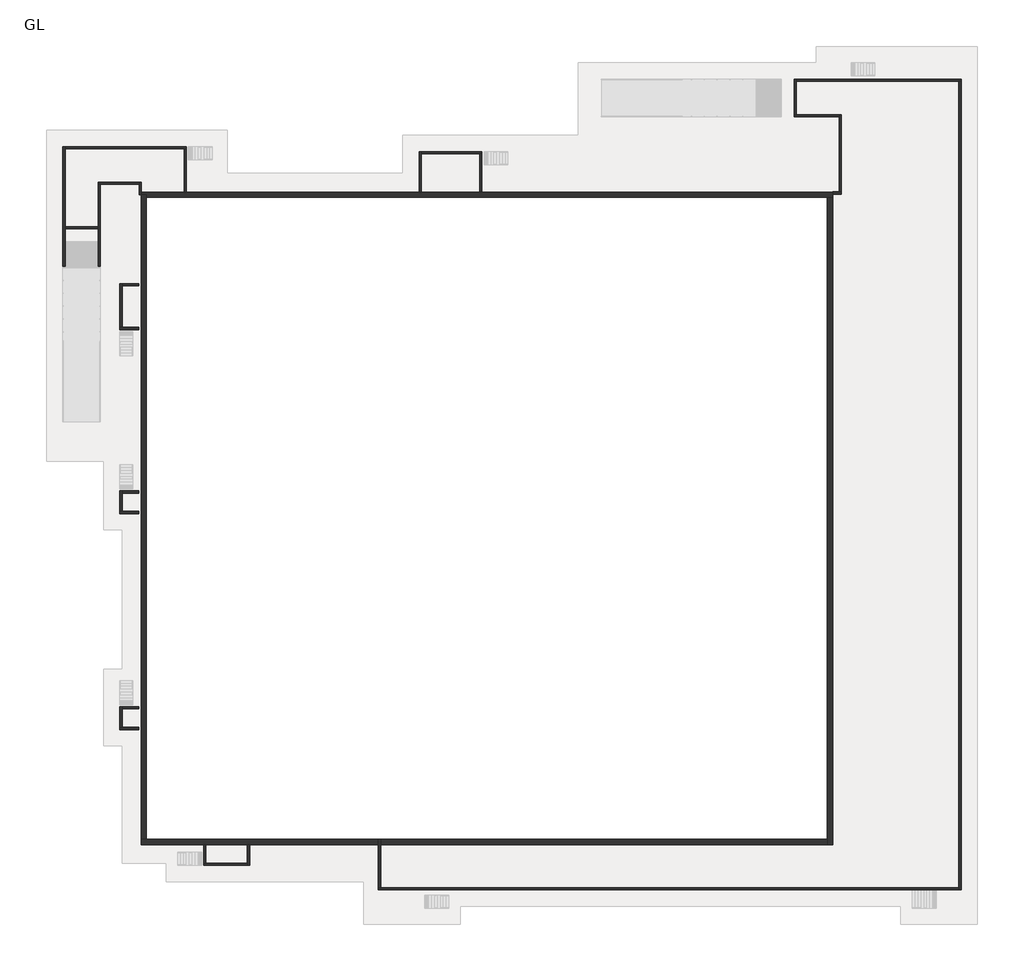
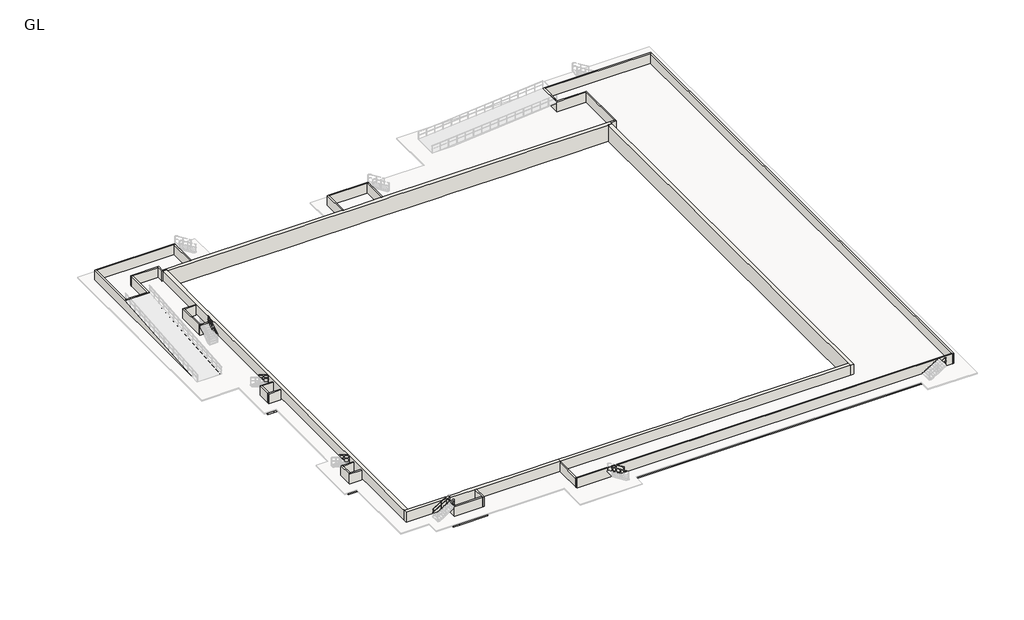
# One storey, part 1 of 2: 35 walls, 22 footings.
"""IFC4 building model written with IfcOpenShell, lengths in millimetres."""

from ifc_helpers import new_model, si_unit, frame, origin, place, context, project, spatial, polyline, outline, extrude, faceted_brep, element, save

model = new_model("IFC4")

# Units and contexts
model_context = context("Model", 3, world=origin())
ifc_project = project(units=[si_unit("LENGTHUNIT", "METRE", prefix="MILLI")], contexts=[model_context])

# Site, building, storey
site = spatial("IfcSite", under=ifc_project)
building = spatial("IfcBuilding", under=site)
storey = spatial("IfcBuildingStorey", under=building, Name="GL", Elevation=-1200.0)

# Footings
placement = place(None, origin())
element("IfcFooting", 1, ObjectType="900x300", at=placement, inside=storey, context=model_context, shape_type="Brep", body=[
    faceted_brep([(-450.0, 11324.7934796, -2200.0), (-450.0, 10424.7934796, -2200.0), (-450.0, 10424.7934796, -2500.0), (-450.0, 11324.7934796, -2500.0), (-1666.0, 11324.7934796, -2200.0), (-2566.0, 11324.7934796, -2200.0), (-2566.0, 10424.7934796, -2200.0), (-2566.0, 10424.7934796, -2500.0), (-2566.0, 11324.7934796, -2500.0), (-1666.0, 11324.7934796, -2500.0)], [[[0, 1, 2, 3]], [[0, 4, 5, 6, 1]], [[2, 1, 6, 7]], [[3, 2, 7, 8, 9]], [[0, 3, 9, 8, 5, 4]], [[6, 5, 8, 7]]]),
])
element("IfcFooting", 2, ObjectType="900x300", at=placement, inside=storey, context=model_context, shape_type="Brep", body=[
    faceted_brep([(-1666.0, 13262.7934796, -2200.0), (-2566.0, 13262.7934796, -2200.0), (-2566.0, 11324.7934796, -2200.0), (-1666.0, 11324.7934796, -2200.0), (-1666.0, 12362.7934796, -2200.0), (-2566.0, 13262.7934796, -2500.0), (-2566.0, 11324.7934796, -2500.0), (-1666.0, 13262.7934796, -2500.0), (-1666.0, 12362.7934796, -2500.0), (-1666.0, 11324.7934796, -2500.0)], [[[0, 1, 2, 3, 4]], [[1, 5, 6, 2]], [[5, 7, 8, 9, 6]], [[7, 0, 4, 3, 9, 8]], [[3, 2, 6, 9]], [[1, 0, 7, 5]]]),
])
element("IfcFooting", 3, ObjectType="900x300", at=placement, inside=storey, context=model_context, shape_type="SweptSolid", body=[
    extrude(outline(polyline([(-450.0, 13262.7934796), (-450.0, 12362.7934796), (-1666.0, 12362.7934796), (-1666.0, 13262.7934796), (-450.0, 13262.7934796)])), frame((0.0, 0.0, -2500.0), z_axis=(0.0, 0.0, 1.0), x_axis=(1.0, 0.0, 0.0)), (0.0, 0.0, 1.0), 300.0),
])
element("IfcFooting", 4, ObjectType="900x300", at=placement, inside=storey, context=model_context, shape_type="Brep", body=[
    faceted_brep([(5264.0, 47.0208589, -2200.0), (6164.0, 47.0208589, -2200.0), (6164.0, 47.0208589, -2500.0), (5264.0, 47.0208589, -2500.0), (6164.0, -2227.9791411, -2200.0), (6164.0, -1327.9791411, -2200.0), (5264.0, -2227.9791411, -2200.0), (5264.0, -2227.9791411, -2500.0), (6164.0, -2227.9791411, -2500.0), (6164.0, -1327.9791411, -2500.0)], [[[0, 1, 2, 3]], [[4, 5, 1, 0, 6]], [[7, 6, 0, 3]], [[8, 7, 3, 2, 9]], [[4, 8, 9, 2, 1, 5]], [[4, 6, 7, 8]]]),
])
element("IfcFooting", 5, ObjectType="900x300", at=placement, inside=storey, context=model_context, shape_type="Brep", body=[
    faceted_brep([(10234.5452414, -2227.9791411, -2200.0), (10234.5452414, -1327.9791411, -2200.0), (9334.5452414, -1327.9791411, -2200.0), (6164.0, -1327.9791411, -2200.0), (6164.0, -2227.9791411, -2200.0), (10234.5452414, -2227.9791411, -2500.0), (6164.0, -2227.9791411, -2500.0), (10234.5452414, -1327.9791411, -2500.0), (6164.0, -1327.9791411, -2500.0), (9334.5452414, -1327.9791411, -2500.0)], [[[0, 1, 2, 3, 4]], [[5, 0, 4, 6]], [[7, 5, 6, 8, 9]], [[1, 7, 9, 8, 3, 2]], [[4, 3, 8, 6]], [[1, 0, 5, 7]]]),
])
element("IfcFooting", 6, ObjectType="900x300", at=placement, inside=storey, context=model_context, shape_type="SweptSolid", body=[
    extrude(outline(polyline([(9334.5452414, 47.0208589), (10234.5452414, 47.0208589), (10234.5452414, -1327.9791411), (9334.5452414, -1327.9791411), (9334.5452414, 47.0208589)])), frame((0.0, 0.0, -2500.0), z_axis=(0.0, 0.0, 1.0), x_axis=(1.0, 0.0, 0.0)), (0.0, 0.0, 1.0), 300.0),
])
element("IfcFooting", 7, ObjectType="900x300", at=placement, inside=storey, context=model_context, shape_type="Brep", body=[
    faceted_brep([(21564.0, 547.0208589, -2200.0), (22464.0, 547.0208589, -2200.0), (22464.0, 547.0208589, -2500.0), (21564.0, 547.0208589, -2500.0), (22464.0, -4527.9791411, -2200.0), (22464.0, -3627.9791411, -2200.0), (21564.0, -4527.9791411, -2200.0), (21564.0, -4527.9791411, -2500.0), (22464.0, -4527.9791411, -2500.0), (22464.0, -3627.9791411, -2500.0)], [[[0, 1, 2, 3]], [[4, 5, 1, 0, 6]], [[7, 6, 0, 3]], [[8, 7, 3, 2, 9]], [[4, 8, 9, 2, 1, 5]], [[4, 6, 7, 8]]]),
])
element("IfcFooting", 8, ObjectType="900x300", at=placement, inside=storey, context=model_context, shape_type="Brep", body=[
    faceted_brep([(76641.0, -4527.9791411, -2200.0), (76641.0, -3627.9791411, -2200.0), (75741.0, -3627.9791411, -2200.0), (22464.0, -3627.9791411, -2200.0), (22464.0, -4527.9791411, -2200.0), (76641.0, -4527.9791411, -2500.0), (22464.0, -4527.9791411, -2500.0), (76641.0, -3627.9791411, -2500.0), (22464.0, -3627.9791411, -2500.0), (75741.0, -3627.9791411, -2500.0)], [[[0, 1, 2, 3, 4]], [[5, 0, 4, 6]], [[7, 5, 6, 8, 9]], [[1, 7, 9, 8, 3, 2]], [[4, 3, 8, 6]], [[1, 0, 5, 7]]]),
])
element("IfcFooting", 9, ObjectType="900x300", at=placement, inside=storey, context=model_context, shape_type="SweptSolid", body=[
    extrude(outline(polyline([(26250.0, 60949.5208589), (25350.0, 60949.5208589), (25350.0, 64152.0208589), (26250.0, 64152.0208589), (26250.0, 60949.5208589)])), frame((0.0, 0.0, -2500.0), z_axis=(0.0, 0.0, 1.0), x_axis=(1.0, 0.0, 0.0)), (0.0, 0.0, 1.0), 300.0),
])
element("IfcFooting", 10, ObjectType="900x300", at=placement, inside=storey, context=model_context, shape_type="Brep", body=[
    faceted_brep([(4325.7243044, 60949.5208589, -2200.0), (3425.7243044, 60949.5208589, -2200.0), (3425.7243044, 60949.5208589, -2500.0), (4325.7243044, 60949.5208589, -2500.0), (3425.7243044, 65527.0208589, -2200.0), (3425.7243044, 64627.0208589, -2200.0), (4325.7243044, 65527.0208589, -2200.0), (4325.7243044, 65527.0208589, -2500.0), (3425.7243044, 65527.0208589, -2500.0), (3425.7243044, 64627.0208589, -2500.0)], [[[0, 1, 2, 3]], [[4, 5, 1, 0, 6]], [[7, 6, 0, 3]], [[8, 7, 3, 2, 9]], [[4, 8, 9, 2, 1, 5]], [[4, 6, 7, 8]]]),
])
element("IfcFooting", 11, ObjectType="900x300", at=placement, inside=storey, context=model_context, shape_type="Brep", body=[
    faceted_brep([(132.1872592, 60699.5208589, -2200.0), (-767.8127408, 60699.5208589, -2200.0), (-767.8127408, 60699.5208589, -2500.0), (132.1872592, 60699.5208589, -2500.0), (132.1872592, 62227.0208589, -2200.0), (-767.8127408, 62227.0208589, -2200.0), (-767.8127408, 61327.0208589, -2200.0), (-767.8127408, 62227.0208589, -2500.0), (-767.8127408, 61327.0208589, -2500.0), (132.1872592, 62227.0208589, -2500.0)], [[[0, 1, 2, 3]], [[0, 4, 5, 6, 1]], [[2, 1, 6, 5, 7, 8]], [[3, 2, 8, 7, 9]], [[0, 3, 9, 4]], [[5, 4, 9, 7]]]),
])
element("IfcFooting", 12, ObjectType="900x300", at=placement, inside=storey, context=model_context, shape_type="Brep", body=[
    faceted_brep([(-4591.0, 62227.0208589, -2200.0), (-4591.0, 61327.0208589, -2200.0), (-3691.0, 61327.0208589, -2200.0), (-767.8127408, 61327.0208589, -2200.0), (-767.8127408, 62227.0208589, -2200.0), (-4591.0, 61327.0208589, -2500.0), (-3691.0, 61327.0208589, -2500.0), (-767.8127408, 61327.0208589, -2500.0), (-4591.0, 62227.0208589, -2500.0), (-767.8127408, 62227.0208589, -2500.0)], [[[0, 1, 2, 3, 4]], [[1, 5, 6, 7, 3, 2]], [[5, 8, 9, 7, 6]], [[8, 0, 4, 9]], [[4, 3, 7, 9]], [[1, 0, 8, 5]]]),
])
element("IfcFooting", 13, ObjectType="900x300", at=placement, inside=storey, context=model_context, shape_type="SweptSolid", body=[
    extrude(outline(polyline([(-7891.0, 64627.0208589), (-7891.0, 65527.0208589), (3425.7243044, 65527.0208589), (3425.7243044, 64627.0208589), (-7891.0, 64627.0208589)])), frame((0.0, 0.0, -2500.0), z_axis=(0.0, 0.0, 1.0), x_axis=(1.0, 0.0, 0.0)), (0.0, 0.0, 1.0), 300.0),
])
element("IfcFooting", 14, ObjectType="900x300", at=placement, inside=storey, context=model_context, shape_type="Brep", body=[
    faceted_brep([(-3691.0, 39561.4815956, -2500.0), (-3691.0, 39561.4815956, -2200.0), (-4591.0, 39561.4815956, -2200.0), (-4591.0, 39561.4815956, -2500.0), (-3691.0, 61327.0208589, -2200.0), (-4591.0, 61327.0208589, -2200.0), (-4591.0, 58048.9598198, -2200.0), (-4591.0, 57148.9598198, -2200.0), (-3691.0, 61327.0208589, -2500.0), (-4591.0, 57148.9598198, -2500.0), (-4591.0, 58048.9598198, -2500.0), (-4591.0, 61327.0208589, -2500.0)], [[[0, 1, 2, 3]], [[2, 1, 4, 5, 6, 7]], [[1, 0, 8, 4]], [[0, 3, 9, 10, 11, 8]], [[3, 2, 7, 6, 5, 11, 10, 9]], [[5, 4, 8, 11]]]),
])
element("IfcFooting", 15, ObjectType="900x300", at=placement, inside=storey, context=model_context, shape_type="Brep", body=[
    faceted_brep([(-6991.0, 39498.9598199, -2200.0), (-7891.0, 39498.9598199, -2200.0), (-7891.0, 39498.9598199, -2500.0), (-6991.0, 39498.9598199, -2500.0), (-6991.0, 57148.9598198, -2200.0), (-6991.0, 58048.9598198, -2200.0), (-6991.0, 64627.0208589, -2200.0), (-7891.0, 65527.0208589, -2200.0), (-7891.0, 65527.0208589, -2500.0), (-6991.0, 64627.0208589, -2500.0), (-6991.0, 58048.9598198, -2500.0), (-6991.0, 57148.9598198, -2500.0)], [[[0, 1, 2, 3]], [[0, 4, 5, 6, 7, 1]], [[2, 1, 7, 8]], [[3, 2, 8, 9, 10, 11]], [[0, 3, 11, 10, 9, 6, 5, 4]], [[7, 6, 9, 8]]]),
    faceted_brep([(-6991.0, 39677.0208589, -2200.0), (-7891.0, 39677.0208589, -2200.0), (-7891.0, 39677.0208589, -2500.0), (-6991.0, 39677.0208589, -2500.0), (-6991.0, 57148.9598198, -2200.0), (-6991.0, 58048.9598198, -2200.0), (-6991.0, 65527.0208589, -2200.0), (-7891.0, 65527.0208589, -2200.0), (-7891.0, 65527.0208589, -2500.0), (-6991.0, 65527.0208589, -2500.0), (-6991.0, 58048.9598198, -2500.0), (-6991.0, 57148.9598198, -2500.0)], [[[0, 1, 2, 3]], [[0, 4, 5, 6, 7, 1]], [[2, 1, 7, 8]], [[3, 2, 8, 9, 10, 11]], [[0, 3, 11, 10, 9, 6, 5, 4]], [[7, 6, 9, 8]]]),
])
element("IfcFooting", 16, ObjectType="900x300", at=placement, inside=storey, context=model_context, shape_type="SweptSolid", body=[
    extrude(outline(polyline([(-4591.0, 58048.9598198), (-4591.0, 57148.9598198), (-6991.0, 57148.9598198), (-6991.0, 58048.9598198), (-4591.0, 58048.9598198)])), frame((0.0, 0.0, -2500.0), z_axis=(0.0, 0.0, 1.0), x_axis=(1.0, 0.0, 0.0)), (0.0, 0.0, 1.0), 300.0),
])
element("IfcFooting", 17, ObjectType="900x300", at=placement, inside=storey, context=model_context, shape_type="Brep", body=[
    faceted_brep([(-450.0, 52734.7934796, -2200.0), (-450.0, 51834.7934796, -2200.0), (-450.0, 51834.7934796, -2500.0), (-450.0, 52734.7934796, -2500.0), (-2566.0, 51834.7934796, -2200.0), (-1666.0, 51834.7934796, -2200.0), (-2566.0, 52734.7934796, -2200.0), (-2566.0, 52734.7934796, -2500.0), (-2566.0, 51834.7934796, -2500.0), (-1666.0, 51834.7934796, -2500.0)], [[[0, 1, 2, 3]], [[4, 5, 1, 0, 6]], [[7, 6, 0, 3]], [[8, 7, 3, 2, 9]], [[4, 8, 9, 2, 1, 5]], [[4, 6, 7, 8]]]),
])
element("IfcFooting", 18, ObjectType="900x300", at=placement, inside=storey, context=model_context, shape_type="Brep", body=[
    faceted_brep([(-2566.0, 47764.2482382, -2200.0), (-1666.0, 47764.2482382, -2200.0), (-1666.0, 48664.2482382, -2200.0), (-1666.0, 51834.7934796, -2200.0), (-2566.0, 51834.7934796, -2200.0), (-2566.0, 47764.2482382, -2500.0), (-2566.0, 51834.7934796, -2500.0), (-1666.0, 47764.2482382, -2500.0), (-1666.0, 51834.7934796, -2500.0), (-1666.0, 48664.2482382, -2500.0)], [[[0, 1, 2, 3, 4]], [[5, 0, 4, 6]], [[7, 5, 6, 8, 9]], [[1, 7, 9, 8, 3, 2]], [[4, 3, 8, 6]], [[1, 0, 5, 7]]]),
])
element("IfcFooting", 19, ObjectType="900x300", at=placement, inside=storey, context=model_context, shape_type="SweptSolid", body=[
    extrude(outline(polyline([(-450.0, 48664.2482382), (-450.0, 47764.2482382), (-1666.0, 47764.2482382), (-1666.0, 48664.2482382), (-450.0, 48664.2482382)])), frame((0.0, 0.0, -2500.0), z_axis=(0.0, 0.0, 1.0), x_axis=(1.0, 0.0, 0.0)), (0.0, 0.0, 1.0), 300.0),
])
element("IfcFooting", 20, ObjectType="900x300", at=placement, inside=storey, context=model_context, shape_type="Brep", body=[
    faceted_brep([(-450.0, 33396.2934796, -2200.0), (-450.0, 32496.2934796, -2200.0), (-450.0, 32496.2934796, -2500.0), (-450.0, 33396.2934796, -2500.0), (-2566.0, 32496.2934796, -2200.0), (-1666.0, 32496.2934796, -2200.0), (-2566.0, 33396.2934796, -2200.0), (-2566.0, 33396.2934796, -2500.0), (-2566.0, 32496.2934796, -2500.0), (-1666.0, 32496.2934796, -2500.0)], [[[0, 1, 2, 3]], [[4, 5, 1, 0, 6]], [[7, 6, 0, 3]], [[8, 7, 3, 2, 9]], [[4, 8, 9, 2, 1, 5]], [[4, 6, 7, 8]]]),
])
element("IfcFooting", 21, ObjectType="900x300", at=placement, inside=storey, context=model_context, shape_type="Brep", body=[
    faceted_brep([(-2566.0, 30586.2934796, -2200.0), (-1666.0, 30586.2934796, -2200.0), (-1666.0, 31486.2934796, -2200.0), (-1666.0, 32496.2934796, -2200.0), (-2566.0, 32496.2934796, -2200.0), (-2566.0, 30586.2934796, -2500.0), (-2566.0, 32496.2934796, -2500.0), (-1666.0, 30586.2934796, -2500.0), (-1666.0, 32496.2934796, -2500.0), (-1666.0, 31486.2934796, -2500.0)], [[[0, 1, 2, 3, 4]], [[5, 0, 4, 6]], [[7, 5, 6, 8, 9]], [[1, 7, 9, 8, 3, 2]], [[4, 3, 8, 6]], [[1, 0, 5, 7]]]),
])
element("IfcFooting", 22, ObjectType="900x300", at=placement, inside=storey, context=model_context, shape_type="SweptSolid", body=[
    extrude(outline(polyline([(-450.0, 31486.2934796), (-450.0, 30586.2934796), (-1666.0, 30586.2934796), (-1666.0, 31486.2934796), (-450.0, 31486.2934796)])), frame((0.0, 0.0, -2500.0), z_axis=(0.0, 0.0, 1.0), x_axis=(1.0, 0.0, 0.0)), (0.0, 0.0, 1.0), 300.0),
])

# Walls
element("IfcWall", 23, ObjectType="H_WA_AMW_RC Wall_T200 (No Finish)", at=placement, inside=storey, context=model_context, shape_type="Brep", body=[
    faceted_brep([(64291.0, 60752.0208589, -2200.0), (65094.3815191, 60752.0208589, -2200.0), (65094.3815191, 60752.0208589, 300.0), (64291.0, 60752.0208589, 300.0), (64291.0, 60952.0208589, -2200.0), (64291.0, 60952.0208589, 300.0), (64894.3815191, 60952.0208589, 300.0), (65094.3815191, 60952.0208589, 300.0), (65094.3815191, 60952.0208589, -2200.0), (64894.3815191, 60952.0208589, -2200.0), (64291.0, 60949.5208589, -2200.0), (64291.0, 60949.5208589, 300.0)], [[[0, 1, 2, 3]], [[4, 5, 6, 7, 8, 9]], [[1, 0, 10, 4, 9, 8]], [[3, 2, 7, 6, 5, 11]], [[2, 1, 8, 7]], [[0, 3, 11, 5, 4, 10]]]),
])
element("IfcWall", 24, ObjectType="H_WA_AMW_RC Wall_T200 (No Finish)", at=placement, inside=storey, context=model_context, shape_type="Brep", body=[
    faceted_brep([(65094.3815191, 60952.0208589, -2200.0), (65094.3815191, 68177.0208589, -2200.0), (65094.3815191, 68177.0208589, 300.0), (65094.3815191, 60952.0208589, 300.0), (64894.3815191, 60952.0208589, -2200.0), (64894.3815191, 60952.0208589, 300.0), (64894.3815191, 67977.0208589, 300.0), (64894.3815191, 68177.0208589, 300.0), (64894.3815191, 68177.0208589, -2200.0), (64894.3815191, 67977.0208589, -2200.0)], [[[0, 1, 2, 3]], [[4, 5, 6, 7, 8, 9]], [[1, 0, 4, 9, 8]], [[3, 2, 7, 6, 5]], [[0, 3, 5, 4]], [[2, 1, 8, 7]]]),
])
element("IfcWall", 25, ObjectType="H_WA_AMW_RC Wall_T200 (No Finish)", at=placement, inside=storey, context=model_context, shape_type="Brep", body=[
    faceted_brep([(64894.3815191, 68177.0208589, -2200.0), (60916.32048, 68177.0208589, -2200.0), (60716.32048, 68177.0208589, -2200.0), (60716.32048, 68177.0208589, 300.0), (60916.32048, 68177.0208589, 300.0), (64894.3815191, 68177.0208589, 300.0), (64894.3815191, 67977.0208589, -2200.0), (64894.3815191, 67977.0208589, 300.0), (60716.32048, 67977.0208589, 300.0), (60716.32048, 67977.0208589, -2200.0)], [[[0, 1, 2, 3, 4, 5]], [[6, 7, 8, 9]], [[2, 1, 0, 6, 9]], [[5, 4, 3, 8, 7]], [[0, 5, 7, 6]], [[3, 2, 9, 8]]]),
])
element("IfcWall", 26, ObjectType="H_WA_AMW_RC Wall_T200 (No Finish)", at=placement, inside=storey, context=model_context, shape_type="Brep", body=[
    faceted_brep([(60916.32048, 68177.0208589, -2200.0), (60916.32048, 71277.0208589, -2200.0), (60916.32048, 71477.0208589, -2200.0), (60916.32048, 71477.0208589, 300.0), (60916.32048, 71277.0208589, 300.0), (60916.32048, 68177.0208589, 300.0), (60716.32048, 68177.0208589, -2200.0), (60716.32048, 68177.0208589, 300.0), (60716.32048, 71477.0208589, 300.0), (60716.32048, 71477.0208589, -2200.0)], [[[0, 1, 2, 3, 4, 5]], [[6, 7, 8, 9]], [[2, 1, 0, 6, 9]], [[5, 4, 3, 8, 7]], [[0, 5, 7, 6]], [[3, 2, 9, 8]]]),
])
element("IfcWall", 27, ObjectType="H_WA_AMW_RC Wall_T200 (No Finish)", at=placement, inside=storey, context=model_context, shape_type="Brep", body=[
    faceted_brep([(60916.32048, 71277.0208589, -2200.0), (76091.0, 71277.0208589, -2200.0), (76291.0, 71277.0208589, -2200.0), (76291.0, 71277.0208589, 300.0), (76091.0, 71277.0208589, 300.0), (60916.32048, 71277.0208589, 300.0), (60916.32048, 71477.0208589, -2200.0), (60916.32048, 71477.0208589, 300.0), (76291.0, 71477.0208589, 300.0), (76291.0, 71477.0208589, -2200.0)], [[[0, 1, 2, 3, 4, 5]], [[6, 7, 8, 9]], [[2, 1, 0, 6, 9]], [[5, 4, 3, 8, 7]], [[0, 5, 7, 6]], [[3, 2, 9, 8]]]),
])
element("IfcWall", 28, ObjectType="H_WA_AMW_RC Wall_T200 (No Finish)", at=placement, inside=storey, context=model_context, shape_type="Brep", body=[
    faceted_brep([(76091.0, 71277.0208589, -2200.0), (76091.0, -3977.9791411, -2200.0), (76091.0, -4177.9791411, -2200.0), (76091.0, -4177.9791411, 300.0), (76091.0, -3977.9791411, 300.0), (76091.0, 71277.0208589, 300.0), (76291.0, 71277.0208589, -2200.0), (76291.0, 71277.0208589, 300.0), (76291.0, -4177.9791411, 300.0), (76291.0, -4177.9791411, -2200.0)], [[[0, 1, 2, 3, 4, 5]], [[6, 7, 8, 9]], [[2, 1, 0, 6, 9]], [[5, 4, 3, 8, 7]], [[0, 5, 7, 6]], [[3, 2, 9, 8]]]),
])
element("IfcWall", 29, ObjectType="H_WA_AMW_RC Wall_T200 (No Finish)", at=placement, inside=storey, context=model_context, shape_type="Brep", body=[
    faceted_brep([(76091.0, -3977.9791411, -2200.0), (22114.0, -3977.9791411, -2200.0), (21914.0, -3977.9791411, -2200.0), (21914.0, -3977.9791411, 150.0), (21914.0, -3977.9791411, 300.0), (76091.0, -3977.9791411, 300.0), (76091.0, -4177.9791411, -2200.0), (76091.0, -4177.9791411, 300.0), (21914.0, -4177.9791411, 300.0), (21914.0, -4177.9791411, -2200.0)], [[[0, 1, 2, 3, 4, 5]], [[6, 7, 8, 9]], [[2, 1, 0, 6, 9]], [[5, 4, 8, 7]], [[4, 3, 2, 9, 8]], [[0, 5, 7, 6]]]),
])
element("IfcWall", 30, ObjectType="H_WA_AMW_RC Wall_T200 (No Finish)", at=placement, inside=storey, context=model_context, shape_type="Brep", body=[
    faceted_brep([(22114.0, -3977.9791411, -2200.0), (22114.0, 49.5208589, -2200.0), (22114.0, 547.0208589, -2200.0), (22114.0, 547.0208589, 150.0), (22114.0, 49.5208589, 150.0), (22114.0, -3977.9791411, 150.0), (21914.0, -3977.9791411, -2200.0), (21914.0, -3977.9791411, 150.0), (21914.0, 47.0208589, 150.0), (21914.0, 547.0208589, 150.0), (21914.0, 547.0208589, -2200.0), (21914.0, 47.0208589, -2200.0), (22014.0, 547.0208589, 150.0)], [[[0, 1, 2, 3, 4, 5]], [[6, 7, 8, 9, 10, 11]], [[2, 1, 0, 6, 11, 10]], [[5, 4, 3, 12, 9, 8, 7]], [[0, 5, 7, 6]], [[3, 2, 10, 9, 12]]]),
])
element("IfcWall", 31, ObjectType="H_WA_AMW_RC Wall_T200 (No Finish)", at=placement, inside=storey, context=model_context, shape_type="Brep", body=[
    faceted_brep([(9684.5452414, 47.0208589, -2200.0), (9684.5452414, -1677.9791411, -2200.0), (9684.5452414, -1877.9791411, -2200.0), (9684.5452414, -1877.9791411, 300.0), (9684.5452414, -1677.9791411, 300.0), (9684.5452414, 47.0208589, 300.0), (9884.5452414, 47.0208589, -2200.0), (9884.5452414, 47.0208589, 300.0), (9884.5452414, -1877.9791411, 300.0), (9884.5452414, -1877.9791411, -2200.0)], [[[0, 1, 2, 3, 4, 5]], [[6, 7, 8, 9]], [[2, 1, 0, 6, 9]], [[5, 4, 3, 8, 7]], [[3, 2, 9, 8]], [[0, 5, 7, 6]]]),
])
element("IfcWall", 32, ObjectType="H_WA_AMW_RC Wall_T200 (No Finish)", at=placement, inside=storey, context=model_context, shape_type="Brep", body=[
    faceted_brep([(9684.5452414, -1677.9791411, -2200.0), (5814.0, -1677.9791411, -2200.0), (5614.0, -1677.9791411, -2200.0), (5614.0, -1677.9791411, 300.0), (5814.0, -1677.9791411, 300.0), (9684.5452414, -1677.9791411, 300.0), (9684.5452414, -1877.9791411, -2200.0), (9684.5452414, -1877.9791411, 300.0), (5614.0, -1877.9791411, 300.0), (5614.0, -1877.9791411, -2200.0)], [[[0, 1, 2, 3, 4, 5]], [[6, 7, 8, 9]], [[2, 1, 0, 6, 9]], [[5, 4, 3, 8, 7]], [[0, 5, 7, 6]], [[3, 2, 9, 8]]]),
])
element("IfcWall", 33, ObjectType="H_WA_AMW_RC Wall_T200 (No Finish)", at=placement, inside=storey, context=model_context, shape_type="SweptSolid", body=[
    extrude(outline(polyline([(5814.0, 47.0208589), (5814.0, -1677.9791411), (5614.0, -1677.9791411), (5614.0, 47.0208589), (5814.0, 47.0208589)])), frame((0.0, 0.0, -2200.0), z_axis=(0.0, 0.0, 1.0), x_axis=(1.0, 0.0, 0.0)), (0.0, 0.0, 1.0), 2500.0),
])
element("IfcWall", 34, ObjectType="H_WA_AMW_RC Wall_T200 (No Finish)", at=placement, inside=storey, context=model_context, shape_type="Brep", body=[
    faceted_brep([(-450.0, 10974.7934796, -2200.0), (-2016.0, 10974.7934796, -2200.0), (-2216.0, 10974.7934796, -2200.0), (-2216.0, 10974.7934796, 300.0), (-2016.0, 10974.7934796, 300.0), (-450.0, 10974.7934796, 300.0), (-450.0, 10774.7934796, -2200.0), (-450.0, 10774.7934796, 300.0), (-2216.0, 10774.7934796, 300.0), (-2216.0, 10774.7934796, -2200.0)], [[[0, 1, 2, 3, 4, 5]], [[6, 7, 8, 9]], [[2, 1, 0, 6, 9]], [[5, 4, 3, 8, 7]], [[0, 5, 7, 6]], [[3, 2, 9, 8]]]),
])
element("IfcWall", 35, ObjectType="H_WA_AMW_RC Wall_T200 (No Finish)", at=placement, inside=storey, context=model_context, shape_type="Brep", body=[
    faceted_brep([(-2016.0, 10974.7934796, -2200.0), (-2016.0, 12712.7934796, -2200.0), (-2016.0, 12912.7934796, -2200.0), (-2016.0, 12912.7934796, 300.0), (-2016.0, 12712.7934796, 300.0), (-2016.0, 10974.7934796, 300.0), (-2216.0, 10974.7934796, -2200.0), (-2216.0, 10974.7934796, 300.0), (-2216.0, 12912.7934796, 300.0), (-2216.0, 12912.7934796, -2200.0)], [[[0, 1, 2, 3, 4, 5]], [[6, 7, 8, 9]], [[2, 1, 0, 6, 9]], [[5, 4, 3, 8, 7]], [[0, 5, 7, 6]], [[3, 2, 9, 8]]]),
])
element("IfcWall", 36, ObjectType="H_WA_AMW_RC Wall_T200 (No Finish)", at=placement, inside=storey, context=model_context, shape_type="SweptSolid", body=[
    extrude(outline(polyline([(-450.0, 12712.7934796), (-2016.0, 12712.7934796), (-2016.0, 12912.7934796), (-450.0, 12912.7934796), (-450.0, 12712.7934796)])), frame((0.0, 0.0, -2200.0), z_axis=(0.0, 0.0, 1.0), x_axis=(1.0, 0.0, 0.0)), (0.0, 0.0, 1.0), 2500.0),
])
element("IfcWall", 37, ObjectType="H_WA_AMW_RC Wall_T200 (No Finish)", at=placement, inside=storey, context=model_context, shape_type="Brep", body=[
    faceted_brep([(-450.0, 31136.2934796, -2200.0), (-2016.0, 31136.2934796, -2200.0), (-2216.0, 31136.2934796, -2200.0), (-2216.0, 31136.2934796, 300.0), (-2016.0, 31136.2934796, 300.0), (-450.0, 31136.2934796, 300.0), (-450.0, 30936.2934796, -2200.0), (-450.0, 30936.2934796, 300.0), (-2216.0, 30936.2934796, 300.0), (-2216.0, 30936.2934796, -2200.0)], [[[0, 1, 2, 3, 4, 5]], [[6, 7, 8, 9]], [[2, 1, 0, 6, 9]], [[5, 4, 3, 8, 7]], [[0, 5, 7, 6]], [[3, 2, 9, 8]]]),
])
element("IfcWall", 38, ObjectType="H_WA_AMW_RC Wall_T200 (No Finish)", at=placement, inside=storey, context=model_context, shape_type="Brep", body=[
    faceted_brep([(-2016.0, 31136.2934796, -2200.0), (-2016.0, 32846.2934796, -2200.0), (-2016.0, 33046.2934796, -2200.0), (-2016.0, 33046.2934796, 300.0), (-2016.0, 32846.2934796, 300.0), (-2016.0, 31136.2934796, 300.0), (-2216.0, 31136.2934796, -2200.0), (-2216.0, 31136.2934796, 300.0), (-2216.0, 33046.2934796, 300.0), (-2216.0, 33046.2934796, -2200.0)], [[[0, 1, 2, 3, 4, 5]], [[6, 7, 8, 9]], [[2, 1, 0, 6, 9]], [[5, 4, 3, 8, 7]], [[0, 5, 7, 6]], [[3, 2, 9, 8]]]),
])
element("IfcWall", 39, ObjectType="H_WA_AMW_RC Wall_T200 (No Finish)", at=placement, inside=storey, context=model_context, shape_type="SweptSolid", body=[
    extrude(outline(polyline([(-450.0, 32846.2934796), (-2016.0, 32846.2934796), (-2016.0, 33046.2934796), (-450.0, 33046.2934796), (-450.0, 32846.2934796)])), frame((0.0, 0.0, -2200.0), z_axis=(0.0, 0.0, 1.0), x_axis=(1.0, 0.0, 0.0)), (0.0, 0.0, 1.0), 2500.0),
])
element("IfcWall", 40, ObjectType="H_WA_AMW_RC Wall_T200 (No Finish)", at=placement, inside=storey, context=model_context, shape_type="Brep", body=[
    faceted_brep([(-450.0, 48314.2482382, -2200.0), (-2016.0, 48314.2482382, -2200.0), (-2216.0, 48314.2482382, -2200.0), (-2216.0, 48314.2482382, 300.0), (-2016.0, 48314.2482382, 300.0), (-450.0, 48314.2482382, 300.0), (-450.0, 48114.2482382, -2200.0), (-450.0, 48114.2482382, 300.0), (-2216.0, 48114.2482382, 300.0), (-2216.0, 48114.2482382, -2200.0)], [[[0, 1, 2, 3, 4, 5]], [[6, 7, 8, 9]], [[2, 1, 0, 6, 9]], [[5, 4, 3, 8, 7]], [[0, 5, 7, 6]], [[3, 2, 9, 8]]]),
])
element("IfcWall", 41, ObjectType="H_WA_AMW_RC Wall_T200 (No Finish)", at=placement, inside=storey, context=model_context, shape_type="Brep", body=[
    faceted_brep([(-2016.0, 48314.2482382, -2200.0), (-2016.0, 52184.7934796, -2200.0), (-2016.0, 52384.7934796, -2200.0), (-2016.0, 52384.7934796, 300.0), (-2016.0, 52184.7934796, 300.0), (-2016.0, 48314.2482382, 300.0), (-2216.0, 48314.2482382, -2200.0), (-2216.0, 48314.2482382, 300.0), (-2216.0, 52384.7934796, 300.0), (-2216.0, 52384.7934796, -2200.0)], [[[0, 1, 2, 3, 4, 5]], [[6, 7, 8, 9]], [[2, 1, 0, 6, 9]], [[5, 4, 3, 8, 7]], [[0, 5, 7, 6]], [[3, 2, 9, 8]]]),
])
element("IfcWall", 42, ObjectType="H_WA_AMW_RC Wall_T200 (No Finish)", at=placement, inside=storey, context=model_context, shape_type="SweptSolid", body=[
    extrude(outline(polyline([(-450.0, 52184.7934796), (-2016.0, 52184.7934796), (-2016.0, 52384.7934796), (-450.0, 52384.7934796), (-450.0, 52184.7934796)])), frame((0.0, 0.0, -2200.0), z_axis=(0.0, 0.0, 1.0), x_axis=(1.0, 0.0, 0.0)), (0.0, 0.0, 1.0), 2500.0),
])
element("IfcWall", 43, ObjectType="H_WA_AMW_RC Wall_T200 (No Finish)", at=placement, inside=storey, context=model_context, shape_type="Brep", body=[
    faceted_brep([(-217.8127408, 60699.5208589, -2200.0), (-217.8127408, 60949.5208589, -2200.0), (-217.8127408, 61877.0208589, -2200.0), (-217.8127408, 61877.0208589, 300.0), (-217.8127408, 60949.5208589, 300.0), (-217.8127408, 60699.5208589, 300.0), (-417.8127408, 60699.5208589, -2200.0), (-417.8127408, 60699.5208589, 300.0), (-417.8127408, 61677.0208589, 300.0), (-417.8127408, 61877.0208589, 300.0), (-417.8127408, 61877.0208589, -2200.0), (-417.8127408, 61677.0208589, -2200.0), (-246.0, 60699.5208589, -2200.0), (-250.0, 60699.5208589, -2200.0), (-250.0, 60699.5208589, 300.0), (-246.0, 60699.5208589, 300.0)], [[[0, 1, 2, 3, 4, 5]], [[6, 7, 8, 9, 10, 11]], [[2, 1, 0, 12, 13, 6, 11, 10]], [[5, 4, 3, 9, 8, 7, 14, 15]], [[0, 5, 15, 14, 7, 6, 13, 12]], [[3, 2, 10, 9]]]),
])
element("IfcWall", 44, ObjectType="H_WA_AMW_RC Wall_T200 (No Finish)", at=placement, inside=storey, context=model_context, shape_type="Brep", body=[
    faceted_brep([(-417.8127408, 61877.0208589, -2200.0), (-4241.0, 61877.0208589, -2200.0), (-4241.0, 61877.0208589, 300.0), (-417.8127408, 61877.0208589, 300.0), (-417.8127408, 61677.0208589, -2200.0), (-417.8127408, 61677.0208589, 300.0), (-4041.0, 61677.0208589, 300.0), (-4241.0, 61677.0208589, 300.0), (-4241.0, 61677.0208589, -2200.0), (-4041.0, 61677.0208589, -2200.0)], [[[0, 1, 2, 3]], [[4, 5, 6, 7, 8, 9]], [[1, 0, 4, 9, 8]], [[3, 2, 7, 6, 5]], [[0, 3, 5, 4]], [[2, 1, 8, 7]]]),
])
element("IfcWall", 45, ObjectType="H_WA_AMW_RC Wall_T200 (No Finish)", at=placement, inside=storey, context=model_context, shape_type="Brep", body=[
    faceted_brep([(-4241.0, 61677.0208589, -2200.0), (-4241.0, 57698.9598198, -2200.0), (-4241.0, 57498.9598198, -2200.0), (-4241.0, 39561.4815956, -2200.0), (-4241.0, 39561.4815956, -1203.1231854), (-4241.0, 57598.9598198, 300.0), (-4241.0, 57698.9598198, 300.0), (-4241.0, 61677.0208589, 300.0), (-4041.0, 61677.0208589, -2200.0), (-4041.0, 61677.0208589, 300.0), (-4041.0, 57598.9598198, 300.0), (-4041.0, 39561.4815956, -1203.1231854), (-4041.0, 39561.4815956, -2200.0)], [[[0, 1, 2, 3, 4, 5, 6, 7]], [[8, 9, 10, 11, 12]], [[0, 7, 9, 8]], [[3, 2, 1, 0, 8, 12]], [[7, 6, 5, 10, 9]], [[4, 3, 12, 11]], [[5, 4, 11, 10]]]),
])
element("IfcWall", 46, ObjectType="H_WA_AMW_RC Wall_T200 (No Finish)", at=placement, inside=storey, context=model_context, shape_type="Brep", body=[
    faceted_brep([(-4241.0, 57698.9598198, 300.0), (-4241.0, 57698.9598198, -2200.0), (-7341.0, 57698.9598198, -2200.0), (-7341.0, 57698.9598198, 300.0), (-4241.0, 57498.9598198, -2200.0), (-4241.0, 57498.9598198, 300.0), (-7341.0, 57498.9598198, 300.0), (-7341.0, 57498.9598198, -2200.0), (-7341.0, 57598.9598198, 300.0), (-4241.0, 57598.9598198, 300.0)], [[[0, 1, 2, 3]], [[4, 5, 6, 7]], [[2, 1, 4, 7]], [[0, 3, 8, 6, 5, 9]], [[3, 2, 7, 6, 8]], [[0, 9, 5, 4, 1]]]),
])
element("IfcWall", 47, ObjectType="H_WA_AMW_RC Wall_T200 (No Finish)", at=placement, inside=storey, context=model_context, shape_type="Brep", body=[
    faceted_brep([(-7341.0, 39498.9598199, -1208.3333333), (-7341.0, 39498.9598199, -2200.0), (-7341.0, 39677.0208589, -2200.0), (-7341.0, 57498.9598198, -2200.0), (-7341.0, 57698.9598198, -2200.0), (-7341.0, 64977.0208589, -2200.0), (-7341.0, 65177.0208589, -2200.0), (-7341.0, 65177.0208589, 300.0), (-7341.0, 64977.0208589, 300.0), (-7341.0, 57698.9598198, 300.0), (-7341.0, 57598.9598198, 300.0), (-7541.0, 39498.9598199, -1208.3333333), (-7541.0, 57598.9598198, 300.0), (-7541.0, 65177.0208589, 300.0), (-7541.0, 65177.0208589, -2200.0), (-7541.0, 39677.0208589, -2200.0), (-7541.0, 39498.9598199, -2200.0)], [[[0, 1, 2, 3, 4, 5, 6, 7, 8, 9, 10]], [[11, 12, 13, 14, 15, 16]], [[7, 6, 14, 13]], [[6, 5, 4, 3, 2, 15, 14]], [[10, 9, 8, 7, 13, 12]], [[0, 10, 12, 11]], [[1, 0, 11, 16]], [[2, 1, 16, 15]]]),
])
element("IfcWall", 48, ObjectType="H_WA_AMW_RC Wall_T200 (No Finish)", at=placement, inside=storey, context=model_context, shape_type="Brep", body=[
    faceted_brep([(-7341.0, 64977.0208589, -2200.0), (3775.7243044, 64977.0208589, -2200.0), (3975.7243044, 64977.0208589, -2200.0), (3975.7243044, 64977.0208589, 300.0), (3775.7243044, 64977.0208589, 300.0), (-7341.0, 64977.0208589, 300.0), (-7341.0, 65177.0208589, -2200.0), (-7341.0, 65177.0208589, 300.0), (3975.7243044, 65177.0208589, 300.0), (3975.7243044, 65177.0208589, -2200.0)], [[[0, 1, 2, 3, 4, 5]], [[6, 7, 8, 9]], [[2, 1, 0, 6, 9]], [[5, 4, 3, 8, 7]], [[0, 5, 7, 6]], [[3, 2, 9, 8]]]),
])
element("IfcWall", 49, ObjectType="H_WA_AMW_RC Wall_T200 (No Finish)", at=placement, inside=storey, context=model_context, shape_type="SweptSolid", body=[
    extrude(outline(polyline([(3775.7243044, 60949.5208589), (3775.7243044, 64977.0208589), (3975.7243044, 64977.0208589), (3975.7243044, 60949.5208589), (3775.7243044, 60949.5208589)])), frame((0.0, 0.0, -2200.0), z_axis=(0.0, 0.0, 1.0), x_axis=(1.0, 0.0, 0.0)), (0.0, 0.0, 1.0), 2500.0),
])
element("IfcWall", 50, ObjectType="H_WA_AMW_RC Wall_T200 (No Finish)", at=placement, inside=storey, context=model_context, shape_type="Brep", body=[
    faceted_brep([(25900.0, 60949.5208589, -2200.0), (25900.0, 64502.0208589, -2200.0), (25900.0, 64702.0208589, -2200.0), (25900.0, 64702.0208589, 300.0), (25900.0, 64502.0208589, 300.0), (25900.0, 60949.5208589, 300.0), (25700.0, 60949.5208589, -2200.0), (25700.0, 60949.5208589, 300.0), (25700.0, 64702.0208589, 300.0), (25700.0, 64702.0208589, -2200.0)], [[[0, 1, 2, 3, 4, 5]], [[6, 7, 8, 9]], [[2, 1, 0, 6, 9]], [[5, 4, 3, 8, 7]], [[3, 2, 9, 8]], [[0, 5, 7, 6]]]),
])
element("IfcWall", 51, ObjectType="H_WA_AMW_RC Wall_T200 (No Finish)", at=placement, inside=storey, context=model_context, shape_type="Brep", body=[
    faceted_brep([(25900.0, 64502.0208589, -2200.0), (31362.1378478, 64502.0208589, -2200.0), (31562.1378478, 64502.0208589, -2200.0), (31562.1378478, 64502.0208589, 300.0), (31362.1378478, 64502.0208589, 300.0), (25900.0, 64502.0208589, 300.0), (25900.0, 64702.0208589, -2200.0), (25900.0, 64702.0208589, 300.0), (31562.1378478, 64702.0208589, 300.0), (31562.1378478, 64702.0208589, -2200.0)], [[[0, 1, 2, 3, 4, 5]], [[6, 7, 8, 9]], [[2, 1, 0, 6, 9]], [[5, 4, 3, 8, 7]], [[0, 5, 7, 6]], [[3, 2, 9, 8]]]),
])
element("IfcWall", 52, ObjectType="H_WA_AMW_RC Wall_T200 (No Finish)", at=placement, inside=storey, context=model_context, shape_type="SweptSolid", body=[
    extrude(outline(polyline([(31362.1378478, 60949.5208589), (31362.1378478, 64502.0208589), (31562.1378478, 64502.0208589), (31562.1378478, 60949.5208589), (31362.1378478, 60949.5208589)])), frame((0.0, 0.0, -2200.0), z_axis=(0.0, 0.0, 1.0), x_axis=(1.0, 0.0, 0.0)), (0.0, 0.0, 1.0), 2500.0),
])
element("IfcWall", 53, ObjectType="H_WA_AMW_RC Wall_T500 (No Finish)", at=placement, inside=storey, context=model_context, shape_type="Brep", body=[
    faceted_brep([(21914.0, 547.0208589, -2200.0), (16250.0, 547.0208589, -2200.0), (15750.0, 547.0208589, -2200.0), (8250.0, 547.0208589, -2200.0), (7750.0, 547.0208589, -2200.0), (254.0, 547.0208589, -2200.0), (-246.0, 547.0208589, -2200.0), (-246.0, 547.0208589, 300.0), (254.0, 547.0208589, 300.0), (7750.0, 547.0208589, 300.0), (8250.0, 547.0208589, 300.0), (15750.0, 547.0208589, 300.0), (16250.0, 547.0208589, 300.0), (22014.0, 547.0208589, 300.0), (22014.0, 547.0208589, 150.0), (21914.0, 547.0208589, 150.0), (21914.0, 47.0208589, -2200.0), (21914.0, 47.0208589, 150.0), (22014.0, 47.0208589, 150.0), (22014.0, 47.0208589, 300.0), (9884.5452414, 47.0208589, 300.0), (9684.5452414, 47.0208589, 300.0), (5814.0, 47.0208589, 300.0), (5614.0, 47.0208589, 300.0), (-246.0, 47.0208589, 300.0), (-246.0, 47.0208589, -2200.0), (5614.0, 47.0208589, -2200.0), (5814.0, 47.0208589, -2200.0), (9684.5452414, 47.0208589, -2200.0), (9884.5452414, 47.0208589, -2200.0), (-246.0, 49.5208589, -2200.0), (-246.0, 49.5208589, 300.0), (22014.0, 49.5208589, 300.0), (22014.0, 49.5208589, 150.0)], [[[0, 1, 2, 3, 4, 5, 6, 7, 8, 9, 10, 11, 12, 13, 14, 15]], [[16, 17, 18, 19, 20, 21, 22, 23, 24, 25, 26, 27, 28, 29]], [[6, 5, 4, 3, 2, 1, 0, 16, 29, 28, 27, 26, 25, 30]], [[13, 12, 11, 10, 9, 8, 7, 31, 24, 23, 22, 21, 20, 19, 32]], [[7, 6, 30, 25, 24, 31]], [[14, 13, 32, 19, 18, 33]], [[14, 33, 18, 17, 15]], [[0, 15, 17, 16]]]),
])
element("IfcWall", 54, ObjectType="H_WA_AMW_RC Wall_T500 (No Finish)", at=placement, inside=storey, context=model_context, shape_type="Brep", body=[
    faceted_brep([(254.0, 547.0208589, -2200.0), (254.0, 10249.5208589, -2200.0), (254.0, 10749.5208589, -2200.0), (254.0, 20249.5208589, -2200.0), (254.0, 20749.5208589, -2200.0), (254.0, 30249.5208589, -2200.0), (254.0, 30749.5208589, -2200.0), (254.0, 40249.5208589, -2200.0), (254.0, 40749.5208589, -2200.0), (254.0, 50249.5208589, -2200.0), (254.0, 50749.5208589, -2200.0), (254.0, 60449.5208589, -2200.0), (254.0, 60699.5208589, -2200.0), (254.0, 60699.5208589, 300.0), (254.0, 60449.5208589, 300.0), (254.0, 50749.5208589, 300.0), (254.0, 50249.5208589, 300.0), (254.0, 40749.5208589, 300.0), (254.0, 40249.5208589, 300.0), (254.0, 30749.5208589, 300.0), (254.0, 30249.5208589, 300.0), (254.0, 20749.5208589, 300.0), (254.0, 20249.5208589, 300.0), (254.0, 10749.5208589, 300.0), (254.0, 10249.5208589, 300.0), (254.0, 547.0208589, 300.0), (-246.0, 547.0208589, -2200.0), (-246.0, 547.0208589, 300.0), (-246.0, 949.5208589, 300.0), (-246.0, 10249.5208589, 300.0), (-246.0, 10749.5208589, 300.0), (-246.0, 20249.5208589, 300.0), (-246.0, 20749.5208589, 300.0), (-246.0, 30249.5208589, 300.0), (-246.0, 30749.5208589, 300.0), (-246.0, 40249.5208589, 300.0), (-246.0, 40749.5208589, 300.0), (-246.0, 50249.5208589, 300.0), (-246.0, 50749.5208589, 300.0), (-246.0, 60049.5208589, 300.0), (-246.0, 60699.5208589, 300.0), (-246.0, 60699.5208589, -2200.0), (-246.0, 60049.5208589, -2200.0), (-246.0, 50749.5208589, -2200.0), (-246.0, 50249.5208589, -2200.0), (-246.0, 40749.5208589, -2200.0), (-246.0, 40249.5208589, -2200.0), (-246.0, 30749.5208589, -2200.0), (-246.0, 30249.5208589, -2200.0), (-246.0, 20749.5208589, -2200.0), (-246.0, 20249.5208589, -2200.0), (-246.0, 10749.5208589, -2200.0), (-246.0, 10249.5208589, -2200.0), (-246.0, 949.5208589, -2200.0), (-217.8127408, 60699.5208589, -2200.0), (-217.8127408, 60699.5208589, 300.0)], [[[0, 1, 2, 3, 4, 5, 6, 7, 8, 9, 10, 11, 12, 13, 14, 15, 16, 17, 18, 19, 20, 21, 22, 23, 24, 25]], [[26, 27, 28, 29, 30, 31, 32, 33, 34, 35, 36, 37, 38, 39, 40, 41, 42, 43, 44, 45, 46, 47, 48, 49, 50, 51, 52, 53]], [[12, 11, 10, 9, 8, 7, 6, 5, 4, 3, 2, 1, 0, 26, 53, 52, 51, 50, 49, 48, 47, 46, 45, 44, 43, 42, 41, 54]], [[13, 12, 54, 41, 40, 55]], [[25, 24, 23, 22, 21, 20, 19, 18, 17, 16, 15, 14, 13, 55, 40, 39, 38, 37, 36, 35, 34, 33, 32, 31, 30, 29, 28, 27]], [[0, 25, 27, 26]]]),
])
element("IfcWall", 55, ObjectType="H_WA_AMW_RC Wall_T500 (No Finish)", at=placement, inside=storey, context=model_context, shape_type="Brep", body=[
    faceted_brep([(254.0, 60449.5208589, -2200.0), (7750.0, 60449.5208589, -2200.0), (8250.0, 60449.5208589, -2200.0), (15750.0, 60449.5208589, -2200.0), (16250.0, 60449.5208589, -2200.0), (23750.0, 60449.5208589, -2200.0), (24250.0, 60449.5208589, -2200.0), (31750.0, 60449.5208589, -2200.0), (32250.0, 60449.5208589, -2200.0), (39750.0, 60449.5208589, -2200.0), (40250.0, 60449.5208589, -2200.0), (47750.0, 60449.5208589, -2200.0), (48250.0, 60449.5208589, -2200.0), (55750.0, 60449.5208589, -2200.0), (56250.0, 60449.5208589, -2200.0), (63750.0, 60449.5208589, -2200.0), (63791.0, 60449.5208589, -2200.0), (64291.0, 60449.5208589, -2200.0), (64291.0, 60449.5208589, 300.0), (63791.0, 60449.5208589, 300.0), (63750.0, 60449.5208589, 300.0), (56250.0, 60449.5208589, 300.0), (55750.0, 60449.5208589, 300.0), (48250.0, 60449.5208589, 300.0), (47750.0, 60449.5208589, 300.0), (40250.0, 60449.5208589, 300.0), (39750.0, 60449.5208589, 300.0), (32250.0, 60449.5208589, 300.0), (31750.0, 60449.5208589, 300.0), (24250.0, 60449.5208589, 300.0), (23750.0, 60449.5208589, 300.0), (16250.0, 60449.5208589, 300.0), (15750.0, 60449.5208589, 300.0), (8250.0, 60449.5208589, 300.0), (7750.0, 60449.5208589, 300.0), (254.0, 60449.5208589, 300.0), (-217.8127408, 60949.5208589, -2200.0), (-217.8127408, 60949.5208589, 300.0), (3775.7243044, 60949.5208589, 300.0), (3975.7243044, 60949.5208589, 300.0), (25700.0, 60949.5208589, 300.0), (25900.0, 60949.5208589, 300.0), (31362.1378478, 60949.5208589, 300.0), (31562.1378478, 60949.5208589, 300.0), (64291.0, 60949.5208589, 300.0), (64291.0, 60949.5208589, -2200.0), (64250.0, 60949.5208589, -2200.0), (63750.0, 60949.5208589, -2200.0), (56250.0, 60949.5208589, -2200.0), (55750.0, 60949.5208589, -2200.0), (48250.0, 60949.5208589, -2200.0), (47750.0, 60949.5208589, -2200.0), (40250.0, 60949.5208589, -2200.0), (39750.0, 60949.5208589, -2200.0), (32250.0, 60949.5208589, -2200.0), (31750.0, 60949.5208589, -2200.0), (31562.1378478, 60949.5208589, -2200.0), (31362.1378478, 60949.5208589, -2200.0), (25900.0, 60949.5208589, -2200.0), (25700.0, 60949.5208589, -2200.0), (24250.0, 60949.5208589, -2200.0), (23750.0, 60949.5208589, -2200.0), (16250.0, 60949.5208589, -2200.0), (15750.0, 60949.5208589, -2200.0), (8250.0, 60949.5208589, -2200.0), (7750.0, 60949.5208589, -2200.0), (3975.7243044, 60949.5208589, -2200.0), (3775.7243044, 60949.5208589, -2200.0), (250.0, 60949.5208589, -2200.0), (254.0, 60699.5208589, -2200.0), (-217.8127408, 60699.5208589, -2200.0), (64291.0, 60752.0208589, -2200.0), (64291.0, 60752.0208589, 300.0), (-217.8127408, 60699.5208589, 300.0), (254.0, 60699.5208589, 300.0), (254.0, 60699.5208589, -300.0155788), (254.0, 60699.5208589, 100.0)], [[[0, 1, 2, 3, 4, 5, 6, 7, 8, 9, 10, 11, 12, 13, 14, 15, 16, 17, 18, 19, 20, 21, 22, 23, 24, 25, 26, 27, 28, 29, 30, 31, 32, 33, 34, 35]], [[36, 37, 38, 39, 40, 41, 42, 43, 44, 45, 46, 47, 48, 49, 50, 51, 52, 53, 54, 55, 56, 57, 58, 59, 60, 61, 62, 63, 64, 65, 66, 67, 68]], [[17, 16, 15, 14, 13, 12, 11, 10, 9, 8, 7, 6, 5, 4, 3, 2, 1, 0, 69, 70, 36, 68, 67, 66, 65, 64, 63, 62, 61, 60, 59, 58, 57, 56, 55, 54, 53, 52, 51, 50, 49, 48, 47, 46, 45, 71]], [[35, 34, 33, 32, 31, 30, 29, 28, 27, 26, 25, 24, 23, 22, 21, 20, 19, 18, 72, 44, 43, 42, 41, 40, 39, 38, 37, 73, 74]], [[74, 73, 70, 69, 75, 76]], [[73, 37, 36, 70]], [[18, 17, 71, 45, 44, 72]], [[0, 35, 74, 76, 75, 69]]]),
])
element("IfcWall", 56, ObjectType="H_WA_AMW_RC Wall_T500 (No Finish)", at=placement, inside=storey, context=model_context, shape_type="Brep", body=[
    faceted_brep([(63791.0, 60449.5208589, -2200.0), (63791.0, 60049.5208589, -2200.0), (63791.0, 50749.5208589, -2200.0), (63791.0, 50249.5208589, -2200.0), (63791.0, 40749.5208589, -2200.0), (63791.0, 40249.5208589, -2200.0), (63791.0, 30749.5208589, -2200.0), (63791.0, 30249.5208589, -2200.0), (63791.0, 20749.5208589, -2200.0), (63791.0, 20249.5208589, -2200.0), (63791.0, 10749.5208589, -2200.0), (63791.0, 10249.5208589, -2200.0), (63791.0, 949.5208589, -2200.0), (63791.0, 549.5208589, -2200.0), (63791.0, 49.5208589, -2200.0), (63791.0, 49.5208589, 300.0), (63791.0, 549.5208589, 300.0), (63791.0, 949.5208589, 300.0), (63791.0, 10249.5208589, 300.0), (63791.0, 10749.5208589, 300.0), (63791.0, 20249.5208589, 300.0), (63791.0, 20749.5208589, 300.0), (63791.0, 30249.5208589, 300.0), (63791.0, 30749.5208589, 300.0), (63791.0, 40249.5208589, 300.0), (63791.0, 40749.5208589, 300.0), (63791.0, 50249.5208589, 300.0), (63791.0, 50749.5208589, 300.0), (63791.0, 60049.5208589, 300.0), (63791.0, 60449.5208589, 300.0), (64291.0, 60449.5208589, -2200.0), (64291.0, 60449.5208589, 300.0), (64291.0, 50749.5208589, 300.0), (64291.0, 50249.5208589, 300.0), (64291.0, 40749.5208589, 300.0), (64291.0, 40249.5208589, 300.0), (64291.0, 30749.5208589, 300.0), (64291.0, 30249.5208589, 300.0), (64291.0, 20749.5208589, 300.0), (64291.0, 20249.5208589, 300.0), (64291.0, 10749.5208589, 300.0), (64291.0, 10249.5208589, 300.0), (64291.0, 49.5208589, 300.0), (64291.0, 49.5208589, -2200.0), (64291.0, 10249.5208589, -2200.0), (64291.0, 10749.5208589, -2200.0), (64291.0, 20249.5208589, -2200.0), (64291.0, 20749.5208589, -2200.0), (64291.0, 30249.5208589, -2200.0), (64291.0, 30749.5208589, -2200.0), (64291.0, 40249.5208589, -2200.0), (64291.0, 40749.5208589, -2200.0), (64291.0, 50249.5208589, -2200.0), (64291.0, 50749.5208589, -2200.0), (64250.0, 49.5208589, -2200.0)], [[[0, 1, 2, 3, 4, 5, 6, 7, 8, 9, 10, 11, 12, 13, 14, 15, 16, 17, 18, 19, 20, 21, 22, 23, 24, 25, 26, 27, 28, 29]], [[30, 31, 32, 33, 34, 35, 36, 37, 38, 39, 40, 41, 42, 43, 44, 45, 46, 47, 48, 49, 50, 51, 52, 53]], [[14, 13, 12, 11, 10, 9, 8, 7, 6, 5, 4, 3, 2, 1, 0, 30, 53, 52, 51, 50, 49, 48, 47, 46, 45, 44, 43, 54]], [[29, 28, 27, 26, 25, 24, 23, 22, 21, 20, 19, 18, 17, 16, 15, 42, 41, 40, 39, 38, 37, 36, 35, 34, 33, 32, 31]], [[15, 14, 54, 43, 42]], [[0, 29, 31, 30]]]),
])
element("IfcWall", 57, ObjectType="H_WA_AMW_RC Wall_T500 (No Finish)", at=placement, inside=storey, context=model_context, shape_type="Brep", body=[
    faceted_brep([(63791.0, 549.5208589, -2200.0), (63750.0, 549.5208589, -2200.0), (56250.0, 549.5208589, -2200.0), (55750.0, 549.5208589, -2200.0), (48250.0, 549.5208589, -2200.0), (47750.0, 549.5208589, -2200.0), (40250.0, 549.5208589, -2200.0), (39750.0, 549.5208589, -2200.0), (32250.0, 549.5208589, -2200.0), (31750.0, 549.5208589, -2200.0), (24250.0, 549.5208589, -2200.0), (23750.0, 549.5208589, -2200.0), (22114.0, 549.5208589, -2200.0), (22114.0, 549.5208589, 150.0), (22014.0, 549.5208589, 150.0), (22014.0, 549.5208589, 300.0), (23750.0, 549.5208589, 300.0), (24250.0, 549.5208589, 300.0), (31750.0, 549.5208589, 300.0), (32250.0, 549.5208589, 300.0), (39750.0, 549.5208589, 300.0), (40250.0, 549.5208589, 300.0), (47750.0, 549.5208589, 300.0), (48250.0, 549.5208589, 300.0), (55750.0, 549.5208589, 300.0), (56250.0, 549.5208589, 300.0), (63750.0, 549.5208589, 300.0), (63791.0, 549.5208589, 300.0), (63791.0, 49.5208589, -2200.0), (63791.0, 49.5208589, 300.0), (22014.0, 49.5208589, 300.0), (22014.0, 49.5208589, 150.0), (22114.0, 49.5208589, 150.0), (22114.0, 49.5208589, -2200.0), (23750.0, 49.5208589, -2200.0), (24250.0, 49.5208589, -2200.0), (31750.0, 49.5208589, -2200.0), (32250.0, 49.5208589, -2200.0), (39750.0, 49.5208589, -2200.0), (40250.0, 49.5208589, -2200.0), (47750.0, 49.5208589, -2200.0), (48250.0, 49.5208589, -2200.0), (55750.0, 49.5208589, -2200.0), (56250.0, 49.5208589, -2200.0), (63750.0, 49.5208589, -2200.0), (22114.0, 547.0208589, -2200.0), (22014.0, 547.0208589, 300.0), (22014.0, 547.0208589, 150.0), (22114.0, 547.0208589, 150.0)], [[[0, 1, 2, 3, 4, 5, 6, 7, 8, 9, 10, 11, 12, 13, 14, 15, 16, 17, 18, 19, 20, 21, 22, 23, 24, 25, 26, 27]], [[28, 29, 30, 31, 32, 33, 34, 35, 36, 37, 38, 39, 40, 41, 42, 43, 44]], [[12, 11, 10, 9, 8, 7, 6, 5, 4, 3, 2, 1, 0, 28, 44, 43, 42, 41, 40, 39, 38, 37, 36, 35, 34, 33, 45]], [[27, 26, 25, 24, 23, 22, 21, 20, 19, 18, 17, 16, 15, 46, 30, 29]], [[0, 27, 29, 28]], [[15, 14, 47, 31, 30, 46]], [[31, 47, 14, 13, 48, 32]], [[13, 12, 45, 33, 32, 48]]]),
])

save(model, "model.ifc")

# Revit data of these elements
# Project information
#   H_Seismic Condition = "A as per ASCE 7-10"
#   H_Soil Condition = "C as per ASCE 7-10"
#   H_Basic Wind Speed = "58.3m/s ASCE7-10"
#   H_DS Project Code = "FAASA2302"
#   H_Project Abbreviation = "SACE2"
#   H_Project Division = "화공"
#   H_Project Finish = "2027-03-05"
#   H_Project Location = "Jafurah, Saudi Arabia"
#   H_Project Start = "2024-01-03"
#   H_Project Type = "EPC"
#   H_Smart Code = "FAASA2302"
#   Project Status = "Project Status"
#   Client Name = "현대엔지니어링"
#   Project Address = "서울시 종로구 율곡로 75(계동)"
#   Project Number = "-"
# Grids (mm)
#   "X1": line (0, 66055.253) -> (0, -2650.221)
#   "X2": line (8000, 66055.253) -> (8000, -2650.221)
#   "Y2": line (-13644.396, 10499.521) -> (72473.433, 10499.521)
#   "Y1": line (-13644.396, 499.521) -> (72473.433, 499.521)
#   "X3": line (16000, 66055.253) -> (16000, -2650.221)
#   "X4": line (24000, 66055.253) -> (24000, -2650.221)
#   "X5": line (32000, 66055.253) -> (32000, -2650.221)
#   "X6": line (40000, 66055.253) -> (40000, -2650.221)
#   "X7": line (48000, 66055.253) -> (48000, -2650.221)
#   "X8": line (56000, 66055.253) -> (56000, -2650.221)
#   "X9": line (64000, 66055.253) -> (64000, -2650.221)
#   "Y3": line (-13644.396, 20499.521) -> (72473.433, 20499.521)
#   "Y4": line (-13644.396, 30499.521) -> (72473.433, 30499.521)
#   "Y5": line (-13644.396, 40499.521) -> (72473.433, 40499.521)
#   "Y6": line (-13644.396, 50499.521) -> (72473.433, 50499.521)
#   "Y7": line (-13644.396, 60499.521) -> (72473.433, 60499.521)
#   "Y8": line (27280.473, 8499.521) -> (-450, 8499.521)
#   "Y9": line (26000, 12805.307) -> (26000, 349.521)
#   "Y10": line (45435.434, 11499.521) -> (25163.697, 11499.521)
#   "Y11": line (44500, -1527.652) -> (44500, 17720.891)
#   "Y12": line (66225.925, 16499.521) -> (42550.657, 16499.521)
#   "Y13": line (33685.38, 47999.521) -> (0, 47999.521)
#   "Y14": line (11500, 57250.62) -> (11500, 48499.521)
#   "Y15": line (26086.356, 55999.521) -> (10701.801, 55999.521)
#   "Y16": line (25500, 61867.552) -> (25500, 49401.462)
#   "Y17": line (27500, 61867.552) -> (27500, 49401.462)
#   "Y19": line (32588.148, 54699.521) -> (27280.473, 54699.521)
#   "Y20": line (16218, 50223.017) -> (16218, 60499.521)
#   "Y21": line (8218, 49.521) -> (8218, 8899.521)
#   "Y24": line (23835, 50223.017) -> (23835, 60499.521)
#   "Y25": line (16218, 49.521) -> (16218, 8899.521)
#   "Y26": line (24218, 49.521) -> (24218, 8899.521)
#   "Y18": line (26086.356, 53249.521) -> (23482.692, 53249.521)
# Type "900x300"
#   Type Comments = "구조_콘크리트"
# Type "H_WA_AMW_RC Wall_T200 (No Finish)"
#   Type Comments = ""
#   Layers, outside or top first: 0 mm no material (function 100); 0 mm no material (function 100); 200 mm no material (function 1); 0 mm no material (function 100); 0 mm no material (function 100); 0 mm no material (function 100)
# Type "H_WA_AMW_RC Wall_T500 (No Finish)"
#   Type Comments = ""
#   Layers, outside or top first: 0 mm no material (function 100); 0 mm no material (function 100); 500 mm no material (function 1); 0 mm no material (function 100); 0 mm no material (function 100); 0 mm no material (function 100)
# Elements 1, 2, 3, 4, 5, 6, 7, 8, 9, 10, 11, 12, 13, 14, 15, 16, 17, 18, 19, 20, 21, 22 (IfcFooting, "900x300")
#   Comments = ""
#   Phase Created = New Construction
# Elements 23, 24, 25, 26, 27, 28, 29, 31, 32, 33, 34, 35, 36, 37, 38, 39, 40, 41, 42, 43, 44, 45, 46, 47, 48, 49, 50, 51, 52 (IfcWall, "H_WA_AMW_RC Wall_T200 (No Finish)")
#   built-in parameter 1001111 = -1000 mm
#   Top Offset = 0 mm
#   Base Offset = -1000 mm
#   wall height = 2500 mm
#   Phase Created = New Construction
#   Base Constraint = GL
#   Top Constraint = FFL
#   Materials on its faces: "Default Wall"
# Element 30 (IfcWall, "H_WA_AMW_RC Wall_T200 (No Finish)")
#   built-in parameter 1001111 = -1000 mm
#   Top Offset = 0 mm
#   Base Offset = -1000 mm
#   wall height = 2350 mm
#   Phase Created = New Construction
#   Base Constraint = GL
#   Top Constraint = FFL
#   Materials on its faces: "Default Wall"
# Elements 53, 54, 55, 56, 57 (IfcWall, "H_WA_AMW_RC Wall_T500 (No Finish)")
#   built-in parameter 1001111 = -1000 mm
#   Top Offset = 0 mm
#   Base Offset = -1000 mm
#   wall height = 2500 mm
#   Phase Created = New Construction
#   Base Constraint = GL
#   Top Constraint = FFL
#   Materials on its faces: "Default Wall"
# Materials
#   "Default Wall": class "Miscellaneous", colour RGB 80 80 80, transparency 0
